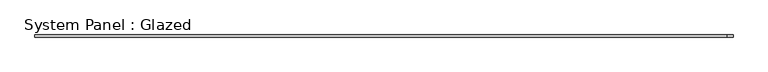
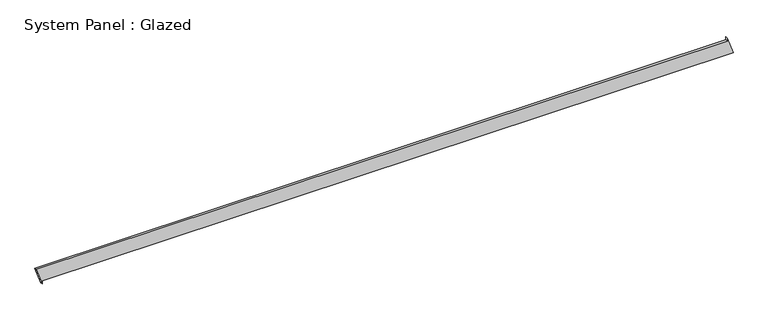
"""IFC4 building model written with IfcOpenShell, lengths in millimetres: plate geometry, System Panel : Glazed."""

from ifc_helpers import new_model, si_unit, frame, origin, place, context, project, spatial, polyline, outline, extrude, source, transform, mapped, element, save


def system_panel_glazed_9d255483(model_context):
    return source(origin(), model_context, "Body", "SweptSolid", [
        extrude(outline(polyline([(0.0, -3958.9104535), (35.3553391, -3958.9104535), (35.3553391, 4027.9323725), (235.7126054, 3959.1507422), (200.3572664, 3959.151181), (200.2581216, -4027.9323725), (0.0, -3958.9104535)])), frame((0.0, -49.5, 0.0), z_axis=(0.0, 1.0, 0.0), x_axis=(0.0, 0.0, 1.0)), (0.0, 0.0, 1.0), 25.0),
    ])


if __name__ == "__main__":
    model = new_model("IFC4")
    model_context = context("Model", 3, world=origin())
    ifc_project = project(units=[si_unit("LENGTHUNIT", "METRE", prefix="MILLI")], contexts=[model_context])
    site = spatial("IfcSite", under=ifc_project)
    building = spatial("IfcBuilding", under=site)
    placement = place(None, origin())
    system_panel_glazed_shape = system_panel_glazed_9d255483(model_context)
    element("IfcPlate", 1, ObjectType="System Panel : Glazed", at=placement, inside=building, context=model_context, shape_type="MappedRepresentation", body=[
        mapped(system_panel_glazed_shape, transform((0.0, 0.0, 0.0), x_axis=(1.0, 0.0, 0.0), y_axis=(0.0, 1.0, 0.0), z_axis=(0.0, 0.0, 1.0))),
    ])
    save(model, "model.ifc")

# Revit data of these elements
# Element 1 (IfcPlate, "System Panel : Glazed")
#   Materials on its faces: "Glass"
# Materials
#   "Glass": class "Glass", colour RGB 218 227 224, transparency 0.85, Description = "Soda Lime Glass", Cost = 0
